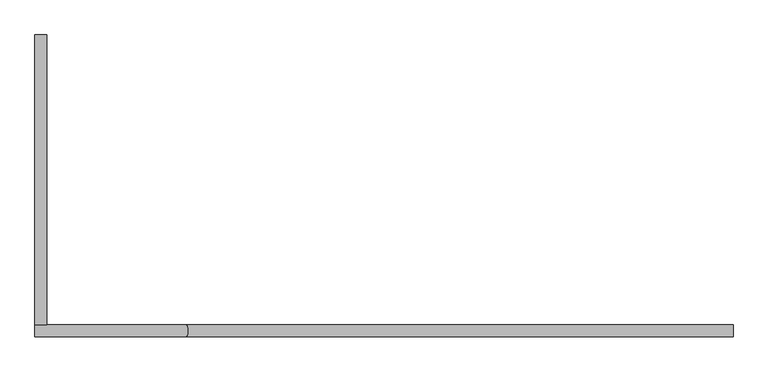
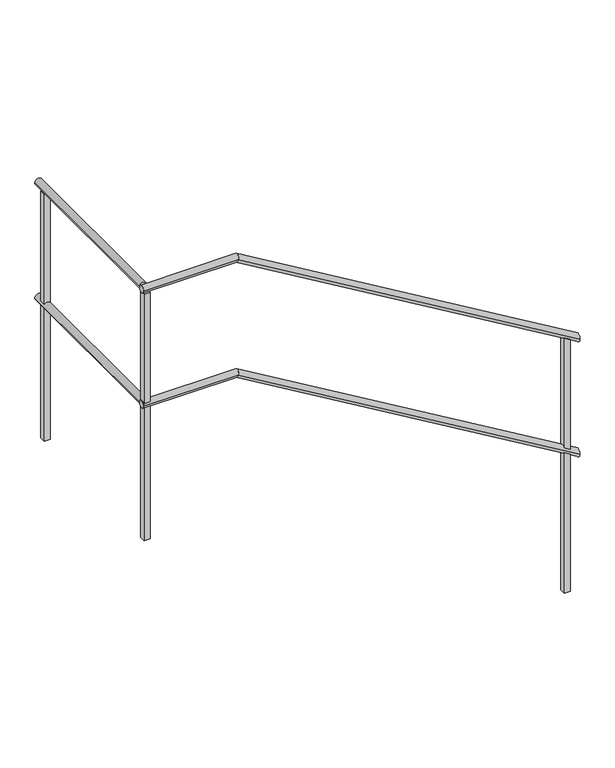
"""IFC4 building model written with IfcOpenShell, lengths in millimetres: railing geometry."""

from ifc_helpers import new_model, si_unit, frame, origin, place, context, project, spatial, polyline, circle_curve, ellipse_curve, outline, extrude, source, transform, mapped, element, save
from ifc_brep_helpers import plane_surface, cylinder_surface, advanced_brep


def railing_cd40e4ad(model_context):
    return source(origin(), model_context, "Body", "SolidModel", [
        advanced_brep(
        [(28067.5161135, 649.5208589, 1584.9618634), (28037.5161135, 649.5208589, 1584.9618634), (28067.5161135, -95.0791411, 1584.9618634), (28037.5161135, -95.0791411, 1584.9618634)],
        [
            (0, 1, circle_curve(frame((28052.5161135, 649.5208589, 1584.9618634), z_axis=(0.0, 1.0, 0.0), x_axis=(-1.0, 0.0, 0.0)), 15.0)),
            (1, 0, circle_curve(frame((28052.5161135, 649.5208589, 1584.9618634), z_axis=(0.0, 1.0, 0.0), x_axis=(-1.0, 0.0, 0.0)), 15.0)),
            (2, 3, circle_curve(frame((28052.5161135, -95.0791411, 1584.9618634), z_axis=(0.0, -1.0, 0.0), x_axis=(-1.0, 0.0, 0.0)), 15.0)),
            (3, 2, circle_curve(frame((28052.5161135, -95.0791411, 1584.9618634), z_axis=(0.0, -1.0, 0.0), x_axis=(-1.0, 0.0, 0.0)), 15.0)),
            (0, 2),
            (3, 1),
        ],
        [
            plane_surface(frame((28052.5161135, 649.5208589, 1599.9618634), z_axis=(0.0, 1.0, 0.0), x_axis=(0.0, 0.0, -1.0))),
            plane_surface(frame((28052.5161135, -95.0791411, 1599.9618634), z_axis=(0.0, -1.0, 0.0), x_axis=(0.0, 0.0, -1.0))),
            cylinder_surface(frame((28052.5161135, 649.5208589, 1584.9618634), z_axis=(0.0, 1.0, 0.0), x_axis=(-1.0, 0.0, 0.0)), 15.0),
        ],
        [
            (0, [[1, 2]]),
            (1, [[3, 4]]),
            (2, [[-1, 5, -4, 6]]),
            (2, [[-2, -6, -3, -5]]),
        ],
    ),
        advanced_brep(
        [(28037.5161135, -95.0791411, 1584.9618634), (28037.5161135, -125.0791411, 1584.9618634), (28425.8735614, -95.0791411, 1584.9618634), (28425.8735614, -125.0791411, 1584.9618634), (29830.0, -95.0791411, 749.1723166), (29830.0, -125.0791411, 749.1723166)],
        [
            (0, 1, circle_curve(frame((28037.5161135, -110.0791411, 1584.9618634), z_axis=(-1.0, 0.0, 0.0), x_axis=(0.0, -1.0, 0.0)), 15.0)),
            (1, 0, circle_curve(frame((28037.5161135, -110.0791411, 1584.9618634), z_axis=(-1.0, 0.0, 0.0), x_axis=(0.0, -1.0, 0.0)), 15.0)),
            (0, 2),
            (2, 3, ellipse_curve(frame((28425.8735614, -110.0791411, 1584.9618634), z_axis=(-0.9641817474962141, 0.0, 0.26524245096731175), x_axis=(-0.26524245096731197, 0.0, -0.964181747496214)), 15.5572329, 15.0)),
            (3, 1),
            (3, 2, ellipse_curve(frame((28425.8735614, -110.0791411, 1584.9618634), z_axis=(-0.9641817474962141, 0.0, 0.26524245096731175), x_axis=(-0.26524245096731197, 0.0, -0.964181747496214)), 15.5572329, 15.0)),
            (4, 5, ellipse_curve(frame((29830.0, -110.0791411, 749.1723166), z_axis=(1.0, 0.0, 0.0), x_axis=(0.0, 0.0, 1.0)), 17.4562134, 15.0)),
            (5, 4, ellipse_curve(frame((29830.0, -110.0791411, 749.1723166), z_axis=(1.0, 0.0, 0.0), x_axis=(0.0, 0.0, 1.0)), 17.4562134, 15.0)),
            (2, 4),
            (5, 3),
        ],
        [
            plane_surface(frame((28037.5161135, -110.0791411, 1599.9618634), z_axis=(-1.0, 0.0, 0.0), x_axis=(0.0, 1.0, 0.0))),
            cylinder_surface(frame((28037.5161135, -110.0791411, 1584.9618634), z_axis=(-1.0, 0.0, 0.0), x_axis=(0.0, -1.0, 0.0)), 15.0),
            plane_surface(frame((29830.0, -110.0791411, 766.62853), z_axis=(1.0, 0.0, 0.0), x_axis=(0.0, 1.0, 0.0))),
            cylinder_surface(frame((28422.3277421, -110.0791411, 1587.0724701), z_axis=(-0.8592928844097064, 0.0, 0.5114838597676831), x_axis=(0.0, -1.0, 0.0)), 15.0),
        ],
        [
            (0, [[1, 2]]),
            (1, [[-1, 3, 4, 5]]),
            (1, [[-2, -5, 6, -3]]),
            (2, [[7, 8]]),
            (3, [[-4, 9, -8, 10]]),
            (3, [[-6, -10, -7, -9]]),
        ],
    ),
        advanced_brep(
        [(28067.5161135, 649.5208589, 2084.9618634), (28037.5161135, 649.5208589, 2084.9618634), (28067.5161135, -95.0791411, 2084.9618634), (28037.5161135, -95.0791411, 2084.9618634)],
        [
            (0, 1, circle_curve(frame((28052.5161135, 649.5208589, 2084.9618634), z_axis=(0.0, 1.0, 0.0), x_axis=(-1.0, 0.0, 0.0)), 15.0)),
            (1, 0, circle_curve(frame((28052.5161135, 649.5208589, 2084.9618634), z_axis=(0.0, 1.0, 0.0), x_axis=(-1.0, 0.0, 0.0)), 15.0)),
            (2, 3, circle_curve(frame((28052.5161135, -95.0791411, 2084.9618634), z_axis=(0.0, -1.0, 0.0), x_axis=(-1.0, 0.0, 0.0)), 15.0)),
            (3, 2, circle_curve(frame((28052.5161135, -95.0791411, 2084.9618634), z_axis=(0.0, -1.0, 0.0), x_axis=(-1.0, 0.0, 0.0)), 15.0)),
            (0, 2),
            (3, 1),
        ],
        [
            plane_surface(frame((28052.5161135, 649.5208589, 2099.9618634), z_axis=(0.0, 1.0, 0.0), x_axis=(0.0, 0.0, -1.0))),
            plane_surface(frame((28052.5161135, -95.0791411, 2099.9618634), z_axis=(0.0, -1.0, 0.0), x_axis=(0.0, 0.0, -1.0))),
            cylinder_surface(frame((28052.5161135, 649.5208589, 2084.9618634), z_axis=(0.0, 1.0, 0.0), x_axis=(-1.0, 0.0, 0.0)), 15.0),
        ],
        [
            (0, [[1, 2]]),
            (1, [[3, 4]]),
            (2, [[-1, 5, -4, 6]]),
            (2, [[-2, -6, -3, -5]]),
        ],
    ),
        advanced_brep(
        [(28037.5161135, -95.0791411, 2084.9618634), (28037.5161135, -125.0791411, 2084.9618634), (28425.8735614, -95.0791411, 2084.9618634), (28425.8735614, -125.0791411, 2084.9618634), (29830.0, -95.0791411, 1249.1723166), (29830.0, -125.0791411, 1249.1723166)],
        [
            (0, 1, circle_curve(frame((28037.5161135, -110.0791411, 2084.9618634), z_axis=(-1.0, 0.0, 0.0), x_axis=(0.0, -1.0, 0.0)), 15.0)),
            (1, 0, circle_curve(frame((28037.5161135, -110.0791411, 2084.9618634), z_axis=(-1.0, 0.0, 0.0), x_axis=(0.0, -1.0, 0.0)), 15.0)),
            (0, 2),
            (2, 3, ellipse_curve(frame((28425.8735614, -110.0791411, 2084.9618634), z_axis=(-0.9641817474962141, 0.0, 0.26524245096731175), x_axis=(-0.26524245096731197, 0.0, -0.964181747496214)), 15.5572329, 15.0)),
            (3, 1),
            (3, 2, ellipse_curve(frame((28425.8735614, -110.0791411, 2084.9618634), z_axis=(-0.9641817474962141, 0.0, 0.26524245096731175), x_axis=(-0.26524245096731197, 0.0, -0.964181747496214)), 15.5572329, 15.0)),
            (4, 5, ellipse_curve(frame((29830.0, -110.0791411, 1249.1723166), z_axis=(1.0, 0.0, 0.0), x_axis=(0.0, 0.0, 1.0)), 17.4562134, 15.0)),
            (5, 4, ellipse_curve(frame((29830.0, -110.0791411, 1249.1723166), z_axis=(1.0, 0.0, 0.0), x_axis=(0.0, 0.0, 1.0)), 17.4562134, 15.0)),
            (2, 4),
            (5, 3),
        ],
        [
            plane_surface(frame((28037.5161135, -110.0791411, 2099.9618634), z_axis=(-1.0, 0.0, 0.0), x_axis=(0.0, 1.0, 0.0))),
            cylinder_surface(frame((28037.5161135, -110.0791411, 2084.9618634), z_axis=(-1.0, 0.0, 0.0), x_axis=(0.0, -1.0, 0.0)), 15.0),
            plane_surface(frame((29830.0, -110.0791411, 1266.62853), z_axis=(1.0, 0.0, 0.0), x_axis=(0.0, 1.0, 0.0))),
            cylinder_surface(frame((28422.3277421, -110.0791411, 2087.0724701), z_axis=(-0.8592928844097064, 0.0, 0.5114838597676831), x_axis=(0.0, -1.0, 0.0)), 15.0),
        ],
        [
            (0, [[1, 2]]),
            (1, [[-1, 3, 4, 5]]),
            (1, [[-2, -5, 6, -3]]),
            (2, [[7, 8]]),
            (3, [[-4, 9, -8, 10]]),
            (3, [[-6, -10, -7, -9]]),
        ],
    ),
        extrude(outline(polyline([(28040.0161135, -97.5791411), (28065.0161135, -97.5791411), (28065.0161135, -122.5791411), (28040.0161135, -122.5791411), (28040.0161135, -97.5791411)])), frame((0.0, 0.0, 999.9618634), z_axis=(0.0, 0.0, 1.0), x_axis=(1.0, 0.0, 0.0)), (0.0, 0.0, 1.0), 1070.0),
        extrude(outline(polyline([(1273.830911, 29767.5), (166.62853, 29767.5), (166.62853, 29792.5), (1258.9499586, 29792.5), (1273.830911, 29767.5)])), frame((0.0, -122.5791411, 0.0), z_axis=(0.0, 1.0, 0.0), x_axis=(0.0, 0.0, 1.0)), (0.0, 0.0, 1.0), 25.0),
        extrude(outline(polyline([(28040.0161135, 612.0208589), (28065.0161135, 612.0208589), (28065.0161135, 587.0208589), (28040.0161135, 587.0208589), (28040.0161135, 612.0208589)])), frame((0.0, 0.0, 999.9618634), z_axis=(0.0, 0.0, 1.0), x_axis=(1.0, 0.0, 0.0)), (0.0, 0.0, 1.0), 1070.0),
    ])


if __name__ == "__main__":
    model = new_model("IFC4")
    model_context = context("Model", 3, world=origin())
    ifc_project = project(units=[si_unit("LENGTHUNIT", "METRE", prefix="MILLI")], contexts=[model_context])
    site = spatial("IfcSite", under=ifc_project)
    building = spatial("IfcBuilding", under=site)
    placement = place(None, origin())
    railing_shape = railing_cd40e4ad(model_context)
    element("IfcRailing", 1, at=placement, inside=building, context=model_context, shape_type="MappedRepresentation", body=[
        mapped(railing_shape, transform((0.0, 0.0, 0.0), x_axis=(1.0, 0.0, 0.0), y_axis=(0.0, 1.0, 0.0), z_axis=(0.0, 0.0, 1.0))),
    ])
    save(model, "model.ifc")
